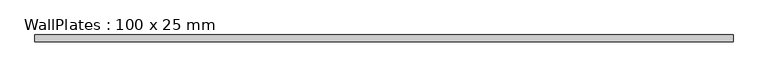
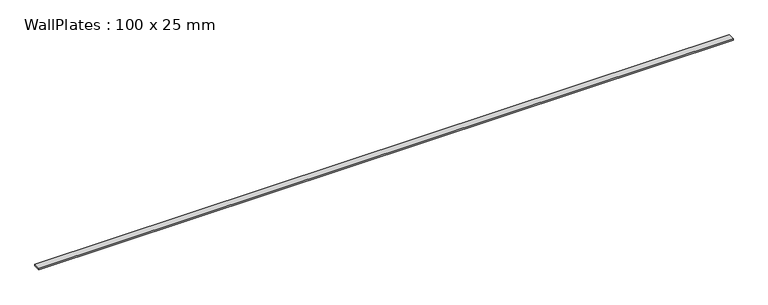
"""IFC4 building model written with IfcOpenShell, lengths in millimetres: beam geometry, WallPlates : 100 x 25 mm."""

from ifc_helpers import new_model, si_unit, frame, origin, place, context, project, spatial, polyline, outline, extrude, source, transform, mapped, element, save


def wallplates_100_x_25_mm_f492c11c(model_context):
    return source(origin(), model_context, "Body", "SweptSolid", [
        extrude(outline(polyline([(-5200.0, -50.0), (-5200.0, 50.0), (5150.0, 50.0), (5150.0, -50.0), (-5200.0, -50.0)])), frame((0.0, 0.0, -12.5), z_axis=(0.0, 0.0, 1.0), x_axis=(1.0, 0.0, 0.0)), (0.0, 0.0, 1.0), 25.0),
    ])


if __name__ == "__main__":
    model = new_model("IFC4")
    model_context = context("Model", 3, world=origin())
    ifc_project = project(units=[si_unit("LENGTHUNIT", "METRE", prefix="MILLI")], contexts=[model_context])
    site = spatial("IfcSite", under=ifc_project)
    building = spatial("IfcBuilding", under=site)
    placement = place(None, origin())
    wallplates_100_x_25_mm_shape = wallplates_100_x_25_mm_f492c11c(model_context)
    element("IfcBeam", 1, ObjectType="WallPlates : 100 x 25 mm", at=placement, inside=building, context=model_context, shape_type="MappedRepresentation", body=[
        mapped(wallplates_100_x_25_mm_shape, transform((0.0, 0.0, 0.0), x_axis=(1.0, 0.0, 0.0), y_axis=(0.0, 1.0, 0.0), z_axis=(0.0, 0.0, 1.0))),
    ])
    save(model, "model.ifc")

# Revit data of these elements
# Type "WallPlates : 100 x 25 mm"
#   ExpertTruss = "Height\th\r\nWidth\tb"
#   Name [instance default] = ""
#   m [instance default] = 0 mm
#   ip_c_cut [instance default] = 1025 mm
#   h_fix [instance default] = 75 mm
#   d/2 [instance default] = 1750 mm
#   c_cut_incl [instance default] = -1000 mm
#   c_cut [instance default] = 0 mm
#   alfaMax [instance default] = 0.00°
#   alfa0_2 [instance default] = 90.00°
#   Alfa_str [instance default] = 0.00°
#   Alfa_cut [instance default] = 90.00°
#   AlfaMAX [instance default] = 0.00°
#   Alfa2_0 [instance default] = 0.00°
#   Alfa2 [instance default] = 0.00°
#   Alfa1_0 [instance default] = 0.00°
#   Alfa1 [instance default] = 0.00°
#   A_max_Str [instance default] = 0.00°
#   h_void [instance default] = 25 mm
#   beam_L_0 [instance default] = 100 mm
#   beam_L [instance default] = 0 mm
#   b_void [instance default] = 110 mm
#   alfa0_1 [instance default] = 90.00°
#   b = 100 mm
#   YOffsetStr [instance default] = 0 mm
#   YOffsetEnd [instance default] = 0 mm
#   XOffsetStr_0 [instance default] = 3500 mm
#   XOffsetStr [instance default] = 0 mm
#   XOffsetEnd_0 [instance default] = 3500 mm
#   XOffsetEnd [instance default] = 0 mm
#   L_void_0 [instance default] = 100 mm
#   L_void [instance default] = 0 mm
#   E2 [instance default] = 0.00°
#   E1 [instance default] = 0.00°
#   Length [instance default] = 3500 mm
#   h = 25 mm
#   Alfa [instance default] = 0.00°
#   A_max_End [instance default] = 0.00°
#   A_max [instance default] = 0.00°
#   A4 [instance default] = 0.00°
#   A3 [instance default] = 0.00°
#   A2 [instance default] = 0.00°
#   A1 [instance default] = 0.00°
#   Material [instance default] = Wood Standard
# Element 1 (IfcBeam, "WallPlates : 100 x 25 mm")
#   d/2 = 5150 mm
#   XOffsetStr_0 = 10350 mm
#   XOffsetStr = -50 mm
#   XOffsetEnd_0 = 10300 mm
#   Materials on its faces: "Wood Standard"
# Materials
#   "Wood Standard": class "Drewno", colour RGB 196 146 67, transparency 0, Cost = 0
